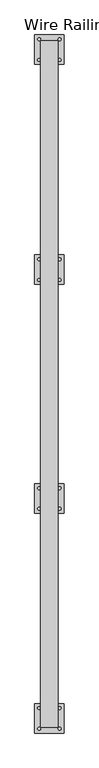
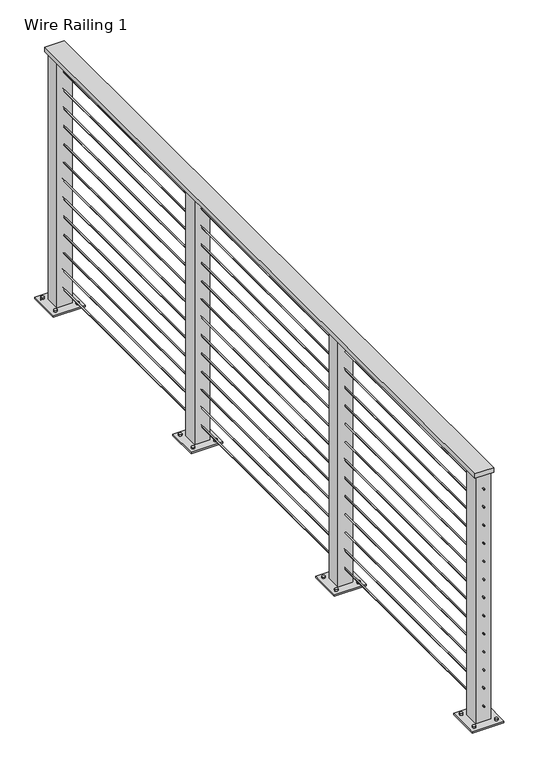
"""IFC4 building model written with IfcOpenShell, lengths in millimetres: railing geometry, Wire Railing 1."""

from ifc_helpers import new_model, si_unit, point, frame, frame_2d, origin, place, context, project, spatial, polyline, circle_curve, trimmed, segment, composite_curve, outline, extrude, source, transform, mapped, element, save


def wire_railing_1_b4026dc2(model_context):
    return source(origin(), model_context, "Body", "SweptSolid", [
        extrude(outline(polyline([(-1874.0398771, -3058.3548735), (-1950.2398771, -3058.3548735), (-1950.2398771, -93.8495308), (-1874.0398771, -93.8495308), (-1874.0398771, -3058.3548735)])), frame((0.0, 0.0, 4502.15), z_axis=(0.0, 0.0, 1.0), x_axis=(1.0, 0.0, 0.0)), (0.0, 0.0, 1.0), 19.05),
        extrude(outline(composite_curve([segment(trimmed(circle_curve(frame_2d((4442.61875, -1912.1398771)), 2.38125), [point((4442.61875, -1909.7586271))], [point((4442.61875, -1914.5211271))], False, "CARTESIAN"), True, "CONTINUOUS"), segment(trimmed(circle_curve(frame_2d((4442.61875, -1912.1398771)), 2.38125), [point((4442.61875, -1914.5211271))], [point((4442.61875, -1909.7586271))], False, "CARTESIAN"), True, "CONTINUOUS")], self_intersect=False)), frame((0.0, -3058.3548735, 0.0), z_axis=(0.0, 1.0, 0.0), x_axis=(0.0, 0.0, 1.0)), (0.0, 0.0, 1.0), 2964.5053427),
        extrude(outline(composite_curve([segment(trimmed(circle_curve(frame_2d((4366.41875, -1912.1398771)), 2.38125), [point((4366.41875, -1909.7586271))], [point((4366.41875, -1914.5211271))], False, "CARTESIAN"), True, "CONTINUOUS"), segment(trimmed(circle_curve(frame_2d((4366.41875, -1912.1398771)), 2.38125), [point((4366.41875, -1914.5211271))], [point((4366.41875, -1909.7586271))], False, "CARTESIAN"), True, "CONTINUOUS")], self_intersect=False)), frame((0.0, -3058.3548735, 0.0), z_axis=(0.0, 1.0, 0.0), x_axis=(0.0, 0.0, 1.0)), (0.0, 0.0, 1.0), 2964.5053427),
        extrude(outline(composite_curve([segment(trimmed(circle_curve(frame_2d((4290.21875, -1912.1398771)), 2.38125), [point((4290.21875, -1909.7586271))], [point((4290.21875, -1914.5211271))], False, "CARTESIAN"), True, "CONTINUOUS"), segment(trimmed(circle_curve(frame_2d((4290.21875, -1912.1398771)), 2.38125), [point((4290.21875, -1914.5211271))], [point((4290.21875, -1909.7586271))], False, "CARTESIAN"), True, "CONTINUOUS")], self_intersect=False)), frame((0.0, -3058.3548735, 0.0), z_axis=(0.0, 1.0, 0.0), x_axis=(0.0, 0.0, 1.0)), (0.0, 0.0, 1.0), 2964.5053427),
        extrude(outline(composite_curve([segment(trimmed(circle_curve(frame_2d((4214.01875, -1912.1398771)), 2.38125), [point((4214.01875, -1909.7586271))], [point((4214.01875, -1914.5211271))], False, "CARTESIAN"), True, "CONTINUOUS"), segment(trimmed(circle_curve(frame_2d((4214.01875, -1912.1398771)), 2.38125), [point((4214.01875, -1914.5211271))], [point((4214.01875, -1909.7586271))], False, "CARTESIAN"), True, "CONTINUOUS")], self_intersect=False)), frame((0.0, -3058.3548735, 0.0), z_axis=(0.0, 1.0, 0.0), x_axis=(0.0, 0.0, 1.0)), (0.0, 0.0, 1.0), 2964.5053427),
        extrude(outline(composite_curve([segment(trimmed(circle_curve(frame_2d((4137.81875, -1912.1398771)), 2.38125), [point((4137.81875, -1909.7586271))], [point((4137.81875, -1914.5211271))], False, "CARTESIAN"), True, "CONTINUOUS"), segment(trimmed(circle_curve(frame_2d((4137.81875, -1912.1398771)), 2.38125), [point((4137.81875, -1914.5211271))], [point((4137.81875, -1909.7586271))], False, "CARTESIAN"), True, "CONTINUOUS")], self_intersect=False)), frame((0.0, -3058.3548735, 0.0), z_axis=(0.0, 1.0, 0.0), x_axis=(0.0, 0.0, 1.0)), (0.0, 0.0, 1.0), 2964.5053427),
        extrude(outline(composite_curve([segment(trimmed(circle_curve(frame_2d((4061.61875, -1912.1398771)), 2.38125), [point((4061.61875, -1909.7586271))], [point((4061.61875, -1914.5211271))], False, "CARTESIAN"), True, "CONTINUOUS"), segment(trimmed(circle_curve(frame_2d((4061.61875, -1912.1398771)), 2.38125), [point((4061.61875, -1914.5211271))], [point((4061.61875, -1909.7586271))], False, "CARTESIAN"), True, "CONTINUOUS")], self_intersect=False)), frame((0.0, -3058.3548735, 0.0), z_axis=(0.0, 1.0, 0.0), x_axis=(0.0, 0.0, 1.0)), (0.0, 0.0, 1.0), 2964.5053427),
        extrude(outline(composite_curve([segment(trimmed(circle_curve(frame_2d((3985.41875, -1912.1398771)), 2.38125), [point((3985.41875, -1909.7586271))], [point((3985.41875, -1914.5211271))], False, "CARTESIAN"), True, "CONTINUOUS"), segment(trimmed(circle_curve(frame_2d((3985.41875, -1912.1398771)), 2.38125), [point((3985.41875, -1914.5211271))], [point((3985.41875, -1909.7586271))], False, "CARTESIAN"), True, "CONTINUOUS")], self_intersect=False)), frame((0.0, -3058.3548735, 0.0), z_axis=(0.0, 1.0, 0.0), x_axis=(0.0, 0.0, 1.0)), (0.0, 0.0, 1.0), 2964.5053427),
        extrude(outline(composite_curve([segment(trimmed(circle_curve(frame_2d((3909.21875, -1912.1398771)), 2.38125), [point((3909.21875, -1909.7586271))], [point((3909.21875, -1914.5211271))], False, "CARTESIAN"), True, "CONTINUOUS"), segment(trimmed(circle_curve(frame_2d((3909.21875, -1912.1398771)), 2.38125), [point((3909.21875, -1914.5211271))], [point((3909.21875, -1909.7586271))], False, "CARTESIAN"), True, "CONTINUOUS")], self_intersect=False)), frame((0.0, -3058.3548735, 0.0), z_axis=(0.0, 1.0, 0.0), x_axis=(0.0, 0.0, 1.0)), (0.0, 0.0, 1.0), 2964.5053427),
        extrude(outline(composite_curve([segment(trimmed(circle_curve(frame_2d((3833.01875, -1912.1398771)), 2.38125), [point((3833.01875, -1909.7586271))], [point((3833.01875, -1914.5211271))], False, "CARTESIAN"), True, "CONTINUOUS"), segment(trimmed(circle_curve(frame_2d((3833.01875, -1912.1398771)), 2.38125), [point((3833.01875, -1914.5211271))], [point((3833.01875, -1909.7586271))], False, "CARTESIAN"), True, "CONTINUOUS")], self_intersect=False)), frame((0.0, -3058.3548735, 0.0), z_axis=(0.0, 1.0, 0.0), x_axis=(0.0, 0.0, 1.0)), (0.0, 0.0, 1.0), 2964.5053427),
        extrude(outline(composite_curve([segment(trimmed(circle_curve(frame_2d((3756.81875, -1912.1398771)), 2.38125), [point((3756.81875, -1909.7586271))], [point((3756.81875, -1914.5211271))], False, "CARTESIAN"), True, "CONTINUOUS"), segment(trimmed(circle_curve(frame_2d((3756.81875, -1912.1398771)), 2.38125), [point((3756.81875, -1914.5211271))], [point((3756.81875, -1909.7586271))], False, "CARTESIAN"), True, "CONTINUOUS")], self_intersect=False)), frame((0.0, -3058.3548735, 0.0), z_axis=(0.0, 1.0, 0.0), x_axis=(0.0, 0.0, 1.0)), (0.0, 0.0, 1.0), 2964.5053427),
        extrude(outline(composite_curve([segment(trimmed(circle_curve(frame_2d((3680.61875, -1912.1398771)), 2.38125), [point((3680.61875, -1909.7586271))], [point((3680.61875, -1914.5211271))], False, "CARTESIAN"), True, "CONTINUOUS"), segment(trimmed(circle_curve(frame_2d((3680.61875, -1912.1398771)), 2.38125), [point((3680.61875, -1914.5211271))], [point((3680.61875, -1909.7586271))], False, "CARTESIAN"), True, "CONTINUOUS")], self_intersect=False)), frame((0.0, -3058.3548735, 0.0), z_axis=(0.0, 1.0, 0.0), x_axis=(0.0, 0.0, 1.0)), (0.0, 0.0, 1.0), 2964.5053427),
        extrude(outline(composite_curve([segment(trimmed(circle_curve(frame_2d((3604.41875, -1912.1398771)), 2.38125), [point((3604.41875, -1909.7586271))], [point((3604.41875, -1914.5211271))], False, "CARTESIAN"), True, "CONTINUOUS"), segment(trimmed(circle_curve(frame_2d((3604.41875, -1912.1398771)), 2.38125), [point((3604.41875, -1914.5211271))], [point((3604.41875, -1909.7586271))], False, "CARTESIAN"), True, "CONTINUOUS")], self_intersect=False)), frame((0.0, -3058.3548735, 0.0), z_axis=(0.0, 1.0, 0.0), x_axis=(0.0, 0.0, 1.0)), (0.0, 0.0, 1.0), 2964.5053427),
        extrude(outline(composite_curve([segment(trimmed(circle_curve(frame_2d((3528.21875, -1912.1398771)), 2.38125), [point((3528.21875, -1909.7586271))], [point((3528.21875, -1914.5211271))], False, "CARTESIAN"), True, "CONTINUOUS"), segment(trimmed(circle_curve(frame_2d((3528.21875, -1912.1398771)), 2.38125), [point((3528.21875, -1914.5211271))], [point((3528.21875, -1909.7586271))], False, "CARTESIAN"), True, "CONTINUOUS")], self_intersect=False)), frame((0.0, -3058.3548735, 0.0), z_axis=(0.0, 1.0, 0.0), x_axis=(0.0, 0.0, 1.0)), (0.0, 0.0, 1.0), 2964.5053427),
        extrude(outline(composite_curve([segment(trimmed(circle_curve(frame_2d((-1956.5898771, -1126.4679784)), 6.35), [point((-1962.9398771, -1126.4679784))], [point((-1950.2398771, -1126.4679784))], False, "CARTESIAN"), True, "CONTINUOUS"), segment(trimmed(circle_curve(frame_2d((-1956.5898771, -1126.4679784)), 6.35), [point((-1950.2398771, -1126.4679784))], [point((-1962.9398771, -1126.4679784))], False, "CARTESIAN"), True, "CONTINUOUS")], self_intersect=False)), frame((0.0, 0.0, 3454.4), z_axis=(0.0, 0.0, 1.0), x_axis=(1.0, 0.0, 0.0)), (0.0, 0.0, 1.0), 12.7),
        extrude(outline(composite_curve([segment(trimmed(circle_curve(frame_2d((-1867.6898771, -1126.4679784)), 6.35), [point((-1874.0398771, -1126.4679784))], [point((-1861.3398771, -1126.4679784))], False, "CARTESIAN"), True, "CONTINUOUS"), segment(trimmed(circle_curve(frame_2d((-1867.6898771, -1126.4679784)), 6.35), [point((-1861.3398771, -1126.4679784))], [point((-1874.0398771, -1126.4679784))], False, "CARTESIAN"), True, "CONTINUOUS")], self_intersect=False)), frame((0.0, 0.0, 3454.4), z_axis=(0.0, 0.0, 1.0), x_axis=(1.0, 0.0, 0.0)), (0.0, 0.0, 1.0), 12.7),
        extrude(outline(composite_curve([segment(trimmed(circle_curve(frame_2d((-1956.5898771, -1037.5679784)), 6.35), [point((-1962.9398771, -1037.5679784))], [point((-1950.2398771, -1037.5679784))], False, "CARTESIAN"), True, "CONTINUOUS"), segment(trimmed(circle_curve(frame_2d((-1956.5898771, -1037.5679784)), 6.35), [point((-1950.2398771, -1037.5679784))], [point((-1962.9398771, -1037.5679784))], False, "CARTESIAN"), True, "CONTINUOUS")], self_intersect=False)), frame((0.0, 0.0, 3454.4), z_axis=(0.0, 0.0, 1.0), x_axis=(1.0, 0.0, 0.0)), (0.0, 0.0, 1.0), 12.7),
        extrude(outline(composite_curve([segment(trimmed(circle_curve(frame_2d((-1867.6898771, -1037.5679784)), 6.35), [point((-1874.0398771, -1037.5679784))], [point((-1861.3398771, -1037.5679784))], False, "CARTESIAN"), True, "CONTINUOUS"), segment(trimmed(circle_curve(frame_2d((-1867.6898771, -1037.5679784)), 6.35), [point((-1861.3398771, -1037.5679784))], [point((-1874.0398771, -1037.5679784))], False, "CARTESIAN"), True, "CONTINUOUS")], self_intersect=False)), frame((0.0, 0.0, 3454.4), z_axis=(0.0, 0.0, 1.0), x_axis=(1.0, 0.0, 0.0)), (0.0, 0.0, 1.0), 12.7),
        extrude(outline(polyline([(-1848.6398771, -1145.5179784), (-1975.6398771, -1145.5179784), (-1975.6398771, -1018.5179784), (-1848.6398771, -1018.5179784), (-1848.6398771, -1145.5179784)])), frame((0.0, 0.0, 3454.4), z_axis=(0.0, 0.0, 1.0), x_axis=(1.0, 0.0, 0.0)), (0.0, 0.0, 1.0), 6.35),
        extrude(outline(polyline([(-1881.9773771, -1112.1804784), (-1942.3023771, -1112.1804784), (-1942.3023771, -1051.8554784), (-1881.9773771, -1051.8554784), (-1881.9773771, -1112.1804784)]), holes=[polyline([(-1888.3273771, -1105.8304784), (-1888.3273771, -1058.2054784), (-1935.9523771, -1058.2054784), (-1935.9523771, -1105.8304784), (-1888.3273771, -1105.8304784)])]), frame((0.0, 0.0, 3454.4), z_axis=(0.0, 0.0, 1.0), x_axis=(1.0, 0.0, 0.0)), (0.0, 0.0, 1.0), 1047.75),
        extrude(outline(composite_curve([segment(trimmed(circle_curve(frame_2d((-1956.5898771, -2114.6364259)), 6.35), [point((-1962.9398771, -2114.6364259))], [point((-1950.2398771, -2114.6364259))], False, "CARTESIAN"), True, "CONTINUOUS"), segment(trimmed(circle_curve(frame_2d((-1956.5898771, -2114.6364259)), 6.35), [point((-1950.2398771, -2114.6364259))], [point((-1962.9398771, -2114.6364259))], False, "CARTESIAN"), True, "CONTINUOUS")], self_intersect=False)), frame((0.0, 0.0, 3454.4), z_axis=(0.0, 0.0, 1.0), x_axis=(1.0, 0.0, 0.0)), (0.0, 0.0, 1.0), 12.7),
        extrude(outline(composite_curve([segment(trimmed(circle_curve(frame_2d((-1867.6898771, -2114.6364259)), 6.35), [point((-1874.0398771, -2114.6364259))], [point((-1861.3398771, -2114.6364259))], False, "CARTESIAN"), True, "CONTINUOUS"), segment(trimmed(circle_curve(frame_2d((-1867.6898771, -2114.6364259)), 6.35), [point((-1861.3398771, -2114.6364259))], [point((-1874.0398771, -2114.6364259))], False, "CARTESIAN"), True, "CONTINUOUS")], self_intersect=False)), frame((0.0, 0.0, 3454.4), z_axis=(0.0, 0.0, 1.0), x_axis=(1.0, 0.0, 0.0)), (0.0, 0.0, 1.0), 12.7),
        extrude(outline(composite_curve([segment(trimmed(circle_curve(frame_2d((-1956.5898771, -2025.7364259)), 6.35), [point((-1962.9398771, -2025.7364259))], [point((-1950.2398771, -2025.7364259))], False, "CARTESIAN"), True, "CONTINUOUS"), segment(trimmed(circle_curve(frame_2d((-1956.5898771, -2025.7364259)), 6.35), [point((-1950.2398771, -2025.7364259))], [point((-1962.9398771, -2025.7364259))], False, "CARTESIAN"), True, "CONTINUOUS")], self_intersect=False)), frame((0.0, 0.0, 3454.4), z_axis=(0.0, 0.0, 1.0), x_axis=(1.0, 0.0, 0.0)), (0.0, 0.0, 1.0), 12.7),
        extrude(outline(composite_curve([segment(trimmed(circle_curve(frame_2d((-1867.6898771, -2025.7364259)), 6.35), [point((-1874.0398771, -2025.7364259))], [point((-1861.3398771, -2025.7364259))], False, "CARTESIAN"), True, "CONTINUOUS"), segment(trimmed(circle_curve(frame_2d((-1867.6898771, -2025.7364259)), 6.35), [point((-1861.3398771, -2025.7364259))], [point((-1874.0398771, -2025.7364259))], False, "CARTESIAN"), True, "CONTINUOUS")], self_intersect=False)), frame((0.0, 0.0, 3454.4), z_axis=(0.0, 0.0, 1.0), x_axis=(1.0, 0.0, 0.0)), (0.0, 0.0, 1.0), 12.7),
        extrude(outline(polyline([(-1848.6398771, -2133.6864259), (-1975.6398771, -2133.6864259), (-1975.6398771, -2006.6864259), (-1848.6398771, -2006.6864259), (-1848.6398771, -2133.6864259)])), frame((0.0, 0.0, 3454.4), z_axis=(0.0, 0.0, 1.0), x_axis=(1.0, 0.0, 0.0)), (0.0, 0.0, 1.0), 6.35),
        extrude(outline(polyline([(-1881.9773771, -2100.3489259), (-1942.3023771, -2100.3489259), (-1942.3023771, -2040.0239259), (-1881.9773771, -2040.0239259), (-1881.9773771, -2100.3489259)]), holes=[polyline([(-1888.3273771, -2093.9989259), (-1888.3273771, -2046.3739259), (-1935.9523771, -2046.3739259), (-1935.9523771, -2093.9989259), (-1888.3273771, -2093.9989259)])]), frame((0.0, 0.0, 3454.4), z_axis=(0.0, 0.0, 1.0), x_axis=(1.0, 0.0, 0.0)), (0.0, 0.0, 1.0), 1047.75),
        extrude(outline(composite_curve([segment(trimmed(circle_curve(frame_2d((-1956.5898771, -176.3995308)), 6.35), [point((-1962.9398771, -176.3995308))], [point((-1950.2398771, -176.3995308))], False, "CARTESIAN"), True, "CONTINUOUS"), segment(trimmed(circle_curve(frame_2d((-1956.5898771, -176.3995308)), 6.35), [point((-1950.2398771, -176.3995308))], [point((-1962.9398771, -176.3995308))], False, "CARTESIAN"), True, "CONTINUOUS")], self_intersect=False)), frame((0.0, 0.0, 3454.4), z_axis=(0.0, 0.0, 1.0), x_axis=(1.0, 0.0, 0.0)), (0.0, 0.0, 1.0), 12.7),
        extrude(outline(composite_curve([segment(trimmed(circle_curve(frame_2d((-1867.6898771, -176.3995308)), 6.35), [point((-1874.0398771, -176.3995308))], [point((-1861.3398771, -176.3995308))], False, "CARTESIAN"), True, "CONTINUOUS"), segment(trimmed(circle_curve(frame_2d((-1867.6898771, -176.3995308)), 6.35), [point((-1861.3398771, -176.3995308))], [point((-1874.0398771, -176.3995308))], False, "CARTESIAN"), True, "CONTINUOUS")], self_intersect=False)), frame((0.0, 0.0, 3454.4), z_axis=(0.0, 0.0, 1.0), x_axis=(1.0, 0.0, 0.0)), (0.0, 0.0, 1.0), 12.7),
        extrude(outline(composite_curve([segment(trimmed(circle_curve(frame_2d((-1956.5898771, -87.4995308)), 6.35), [point((-1962.9398771, -87.4995308))], [point((-1950.2398771, -87.4995308))], False, "CARTESIAN"), True, "CONTINUOUS"), segment(trimmed(circle_curve(frame_2d((-1956.5898771, -87.4995308)), 6.35), [point((-1950.2398771, -87.4995308))], [point((-1962.9398771, -87.4995308))], False, "CARTESIAN"), True, "CONTINUOUS")], self_intersect=False)), frame((0.0, 0.0, 3454.4), z_axis=(0.0, 0.0, 1.0), x_axis=(1.0, 0.0, 0.0)), (0.0, 0.0, 1.0), 12.7),
        extrude(outline(composite_curve([segment(trimmed(circle_curve(frame_2d((-1867.6898771, -87.4995308)), 6.35), [point((-1874.0398771, -87.4995308))], [point((-1861.3398771, -87.4995308))], False, "CARTESIAN"), True, "CONTINUOUS"), segment(trimmed(circle_curve(frame_2d((-1867.6898771, -87.4995308)), 6.35), [point((-1861.3398771, -87.4995308))], [point((-1874.0398771, -87.4995308))], False, "CARTESIAN"), True, "CONTINUOUS")], self_intersect=False)), frame((0.0, 0.0, 3454.4), z_axis=(0.0, 0.0, 1.0), x_axis=(1.0, 0.0, 0.0)), (0.0, 0.0, 1.0), 12.7),
        extrude(outline(polyline([(-1848.6398771, -195.4495308), (-1975.6398771, -195.4495308), (-1975.6398771, -68.4495308), (-1848.6398771, -68.4495308), (-1848.6398771, -195.4495308)])), frame((0.0, 0.0, 3454.4), z_axis=(0.0, 0.0, 1.0), x_axis=(1.0, 0.0, 0.0)), (0.0, 0.0, 1.0), 6.35),
        extrude(outline(polyline([(-1881.9773771, -162.1120308), (-1942.3023771, -162.1120308), (-1942.3023771, -101.7870308), (-1881.9773771, -101.7870308), (-1881.9773771, -162.1120308)]), holes=[polyline([(-1888.3273771, -155.7620308), (-1888.3273771, -108.1370308), (-1935.9523771, -108.1370308), (-1935.9523771, -155.7620308), (-1888.3273771, -155.7620308)])]), frame((0.0, 0.0, 3454.4), z_axis=(0.0, 0.0, 1.0), x_axis=(1.0, 0.0, 0.0)), (0.0, 0.0, 1.0), 1047.75),
        extrude(outline(composite_curve([segment(trimmed(circle_curve(frame_2d((-1956.5898771, -3064.7048735)), 6.35), [point((-1962.9398771, -3064.7048735))], [point((-1950.2398771, -3064.7048735))], False, "CARTESIAN"), True, "CONTINUOUS"), segment(trimmed(circle_curve(frame_2d((-1956.5898771, -3064.7048735)), 6.35), [point((-1950.2398771, -3064.7048735))], [point((-1962.9398771, -3064.7048735))], False, "CARTESIAN"), True, "CONTINUOUS")], self_intersect=False)), frame((0.0, 0.0, 3454.4), z_axis=(0.0, 0.0, 1.0), x_axis=(1.0, 0.0, 0.0)), (0.0, 0.0, 1.0), 12.7),
        extrude(outline(composite_curve([segment(trimmed(circle_curve(frame_2d((-1867.6898771, -3064.7048735)), 6.35), [point((-1874.0398771, -3064.7048735))], [point((-1861.3398771, -3064.7048735))], False, "CARTESIAN"), True, "CONTINUOUS"), segment(trimmed(circle_curve(frame_2d((-1867.6898771, -3064.7048735)), 6.35), [point((-1861.3398771, -3064.7048735))], [point((-1874.0398771, -3064.7048735))], False, "CARTESIAN"), True, "CONTINUOUS")], self_intersect=False)), frame((0.0, 0.0, 3454.4), z_axis=(0.0, 0.0, 1.0), x_axis=(1.0, 0.0, 0.0)), (0.0, 0.0, 1.0), 12.7),
        extrude(outline(composite_curve([segment(trimmed(circle_curve(frame_2d((-1956.5898771, -2975.8048735)), 6.35), [point((-1962.9398771, -2975.8048735))], [point((-1950.2398771, -2975.8048735))], False, "CARTESIAN"), True, "CONTINUOUS"), segment(trimmed(circle_curve(frame_2d((-1956.5898771, -2975.8048735)), 6.35), [point((-1950.2398771, -2975.8048735))], [point((-1962.9398771, -2975.8048735))], False, "CARTESIAN"), True, "CONTINUOUS")], self_intersect=False)), frame((0.0, 0.0, 3454.4), z_axis=(0.0, 0.0, 1.0), x_axis=(1.0, 0.0, 0.0)), (0.0, 0.0, 1.0), 12.7),
        extrude(outline(composite_curve([segment(trimmed(circle_curve(frame_2d((-1867.6898771, -2975.8048735)), 6.35), [point((-1874.0398771, -2975.8048735))], [point((-1861.3398771, -2975.8048735))], False, "CARTESIAN"), True, "CONTINUOUS"), segment(trimmed(circle_curve(frame_2d((-1867.6898771, -2975.8048735)), 6.35), [point((-1861.3398771, -2975.8048735))], [point((-1874.0398771, -2975.8048735))], False, "CARTESIAN"), True, "CONTINUOUS")], self_intersect=False)), frame((0.0, 0.0, 3454.4), z_axis=(0.0, 0.0, 1.0), x_axis=(1.0, 0.0, 0.0)), (0.0, 0.0, 1.0), 12.7),
        extrude(outline(polyline([(-1848.6398771, -3083.7548735), (-1975.6398771, -3083.7548735), (-1975.6398771, -2956.7548735), (-1848.6398771, -2956.7548735), (-1848.6398771, -3083.7548735)])), frame((0.0, 0.0, 3454.4), z_axis=(0.0, 0.0, 1.0), x_axis=(1.0, 0.0, 0.0)), (0.0, 0.0, 1.0), 6.35),
        extrude(outline(polyline([(-1881.9773771, -3050.4173735), (-1942.3023771, -3050.4173735), (-1942.3023771, -2990.0923735), (-1881.9773771, -2990.0923735), (-1881.9773771, -3050.4173735)]), holes=[polyline([(-1888.3273771, -3044.0673735), (-1888.3273771, -2996.4423735), (-1935.9523771, -2996.4423735), (-1935.9523771, -3044.0673735), (-1888.3273771, -3044.0673735)])]), frame((0.0, 0.0, 3454.4), z_axis=(0.0, 0.0, 1.0), x_axis=(1.0, 0.0, 0.0)), (0.0, 0.0, 1.0), 1047.75),
    ])


if __name__ == "__main__":
    model = new_model("IFC4")
    model_context = context("Model", 3, world=origin())
    ifc_project = project(units=[si_unit("LENGTHUNIT", "METRE", prefix="MILLI")], contexts=[model_context])
    site = spatial("IfcSite", under=ifc_project)
    building = spatial("IfcBuilding", under=site)
    placement = place(None, origin())
    wire_railing_1_shape = wire_railing_1_b4026dc2(model_context)
    element("IfcRailing", 1, ObjectType="Wire Railing 1", at=placement, inside=building, context=model_context, shape_type="MappedRepresentation", body=[
        mapped(wire_railing_1_shape, transform((0.0, 0.0, 0.0), x_axis=(1.0, 0.0, 0.0), y_axis=(0.0, 1.0, 0.0), z_axis=(0.0, 0.0, 1.0))),
    ])
    save(model, "model.ifc")

# Revit data of these elements
# Element 1 (IfcRailing, "Wire Railing 1")
#   Materials on its faces: "Metal - Kawneer - Aluminum"
# Materials
#   "Metal - Kawneer - Aluminum": class "Metal", colour RGB 244 244 244, transparency 0, Manufacturer = "Kawneer", URL = "http://www.kawneer.com/kawneer/north_america/en/home.asp", Cost = 0
